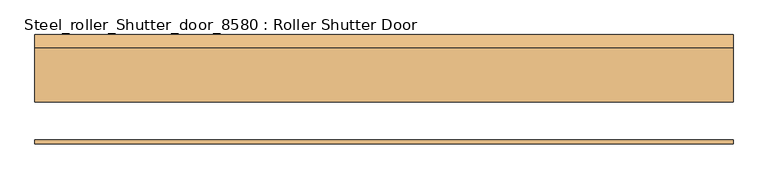
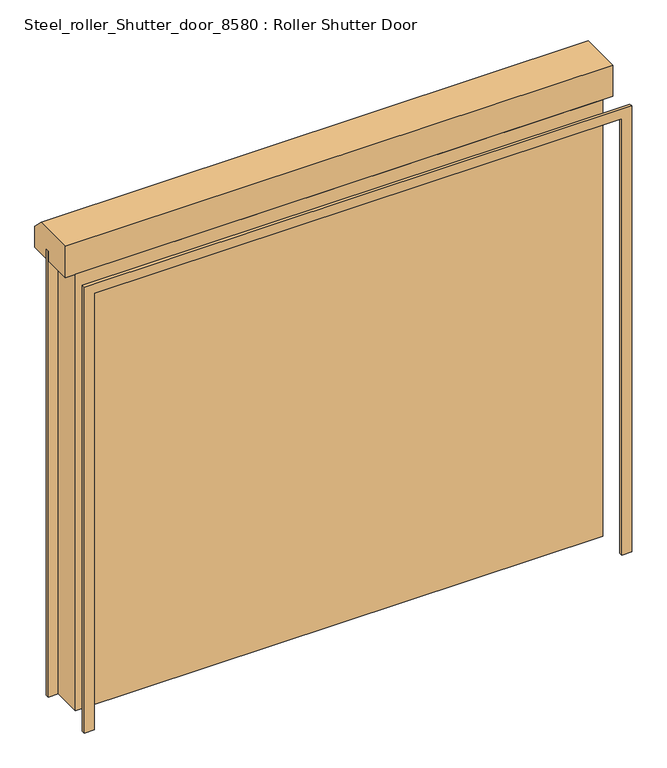
"""IFC4 building model written with IfcOpenShell, lengths in millimetres: door geometry, Steel_roller_Shutter_door_8580 : Roller Shutter Door."""

from ifc_helpers import new_model, si_unit, frame, origin, place, context, project, spatial, polyline, outline, extrude, source, transform, mapped, element, save


def steel_roller_shutter_door_8580_roller_shutter_door_53e56a6d(model_context):
    return source(origin(), model_context, "Body", "SweptSolid", [
        extrude(outline(polyline([(3500.0, -2000.0), (3500.0, 2000.0), (0.0, 2000.0), (0.0, 2075.0), (3575.0, 2075.0), (3575.0, -2075.0), (0.0, -2075.0), (0.0, -2000.0), (3500.0, -2000.0)])), frame((0.0, 225.0, 0.0), z_axis=(0.0, 1.0, 0.0), x_axis=(0.0, 0.0, 1.0)), (0.0, 0.0, 1.0), 25.0),
        extrude(outline(polyline([(3575.0, -2075.0), (0.0, -2075.0), (0.0, -2000.0), (3500.0, -2000.0), (3500.0, 2000.0), (0.0, 2000.0), (0.0, 2075.0), (3575.0, 2075.0), (3575.0, -2075.0)])), frame((0.0, -250.0, 0.0), z_axis=(0.0, 1.0, 0.0), x_axis=(0.0, 0.0, 1.0)), (0.0, 0.0, 1.0), 25.0),
        extrude(outline(polyline([(0.0, 3500.0), (225.0, 3500.0), (225.0, 3475.0), (250.0, 3475.0), (250.0, 0.0), (0.0, 0.0), (0.0, 3500.0)])), frame((-2000.0, 0.0, 0.0), z_axis=(1.0, 0.0, 0.0), x_axis=(0.0, 1.0, 0.0)), (0.0, 0.0, 1.0), 4000.0),
        extrude(outline(polyline([(0.0, 3750.0), (320.0, 3750.0), (400.0, 3670.0), (400.0, 3500.0), (0.0, 3500.0), (0.0, 3750.0)])), frame((-2075.0, 0.0, 0.0), z_axis=(1.0, 0.0, 0.0), x_axis=(0.0, 1.0, 0.0)), (0.0, 0.0, 1.0), 4150.0),
    ])


if __name__ == "__main__":
    model = new_model("IFC4")
    model_context = context("Model", 3, world=origin())
    ifc_project = project(units=[si_unit("LENGTHUNIT", "METRE", prefix="MILLI")], contexts=[model_context])
    site = spatial("IfcSite", under=ifc_project)
    building = spatial("IfcBuilding", under=site)
    placement = place(None, origin())
    steel_roller_shutter_door_8580_roller_shutter_door_shape = steel_roller_shutter_door_8580_roller_shutter_door_53e56a6d(model_context)
    element("IfcDoor", 1, ObjectType="Steel_roller_Shutter_door_8580 : Roller Shutter Door", at=placement, inside=building, context=model_context, shape_type="MappedRepresentation", body=[
        mapped(steel_roller_shutter_door_8580_roller_shutter_door_shape, transform((0.0, 0.0, 0.0), x_axis=(1.0, 0.0, 0.0), y_axis=(0.0, 1.0, 0.0), z_axis=(0.0, 0.0, 1.0))),
    ])
    save(model, "model.ifc")

# Revit data of these elements
# Type "Steel_roller_Shutter_door_8580 : Roller Shutter Door"
#   Type Mark = "36"
#   Frame Projection Ext. = 25 mm
#   Frame Projection Int. = 25 mm
#   Frame Width = 75 mm
#   Height = 3500 mm
#   Width = 4000 mm
#   Function = (empty or 0)
#   Wall Closure = (empty or 0)
#   Assembly Code = ""
# Element 1 (IfcDoor, "Steel_roller_Shutter_door_8580 : Roller Shutter Door")
#   Materials on its faces: "Steel Shutters", "Render 0-255-0"
# Materials
#   "Steel Shutters": class "Vinyl", colour RGB 122 127 125, transparency 0
#   "Render 0-255-0": class "Miscellaneous", colour RGB 0 255 0, transparency 0
